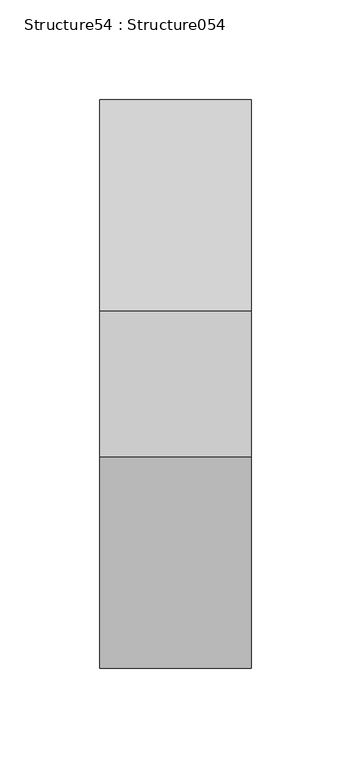
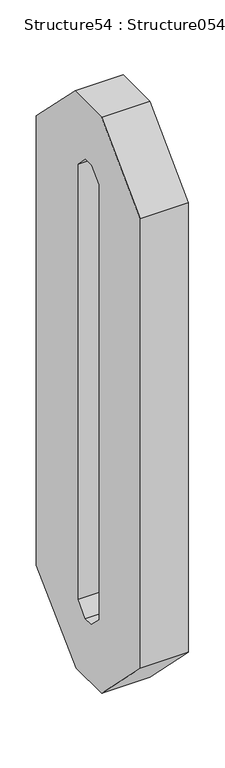
"""IFC4 building model written with IfcOpenShell, lengths in millimetres: proxy geometry, Structure54 : Structure054."""

from ifc_helpers import new_model, si_unit, frame, origin, place, context, project, spatial, polyline, outline, extrude, source, transform, mapped, element, save


def structure54_structure054_f67f94a8(model_context):
    return source(origin(), model_context, "Body", "SweptSolid", [
        extrude(outline(polyline([(249027.9512073, 4382.5453733), (249134.0171383, 4488.6115703), (249207.4507409, 4488.6115703), (249313.5166718, 4382.5456393), (249313.5154123, 3629.2065158), (249203.5119524, 3523.2149577), (249134.0171383, 3523.1417985), (249027.9512073, 3629.2077294), (249027.9512073, 4382.5453733)]), holes=[polyline([(249178.8931238, 3621.0476006), (249199.2918716, 3641.4461544), (249199.2918716, 4370.299463), (249178.8937536, 4390.697581), (249162.5785341, 4390.697581), (249142.1804161, 4370.299463), (249142.1804161, 3641.4463659), (249162.5785341, 3621.0482303), (249178.8931238, 3621.0476006)])]), frame((-38594.2176606, 0.0, 0.0), z_axis=(1.0, 0.0, 0.0), x_axis=(0.0, 1.0, 0.0)), (0.0, 0.0, 1.0), 76.2),
    ])


if __name__ == "__main__":
    model = new_model("IFC4")
    model_context = context("Model", 3, world=origin())
    ifc_project = project(units=[si_unit("LENGTHUNIT", "METRE", prefix="MILLI")], contexts=[model_context])
    site = spatial("IfcSite", under=ifc_project)
    building = spatial("IfcBuilding", under=site)
    placement = place(None, origin())
    structure54_structure054_shape = structure54_structure054_f67f94a8(model_context)
    element("IfcBuildingElementProxy", 1, Name="Structure54 : Structure054", ObjectType="Structure54 : Structure054", at=placement, inside=building, context=model_context, shape_type="MappedRepresentation", body=[
        mapped(structure54_structure054_shape, transform((0.0, 0.0, 0.0), x_axis=(1.0, 0.0, 0.0), y_axis=(0.0, 1.0, 0.0), z_axis=(0.0, 0.0, 1.0))),
    ])
    save(model, "model.ifc")

# Revit data of these elements
# Type "Structure54 : Structure054"
#   NameOverride = "Structure054"
# Element 1 (IfcBuildingElementProxy, "Structure54 : Structure054")
#   Materials on its faces: "BRUSHED ALUM. LETTERING"
# Materials
#   "BRUSHED ALUM. LETTERING": class "Unassigned", colour RGB 169 181 186, transparency 0, Cost = 0
